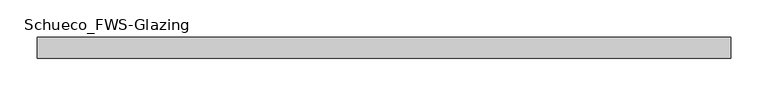
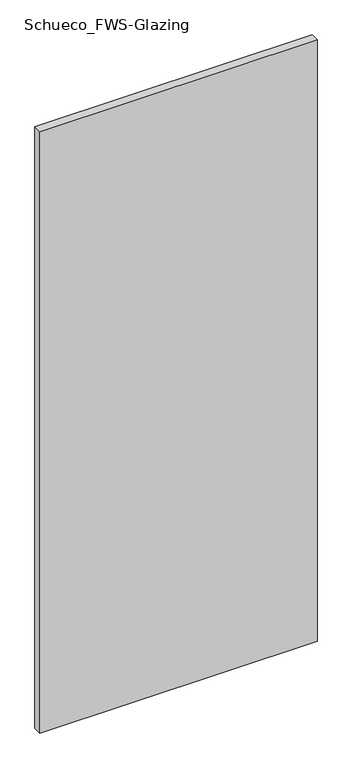
"""IFC4 building model written with IfcOpenShell, lengths in millimetres: plate geometry, Schueco_FWS-Glazing : HI_28mm_DoubGlz."""

from ifc_helpers import new_model, si_unit, origin, origin_with_axes, place, context, project, spatial, polyline, outline, extrude, source, transform, mapped, element, save


def schueco_fws_glazing_3bf565c2(model_context):
    return source(origin(), model_context, "Body", "SweptSolid", [
        extrude(outline(polyline([(464.0, -28.0), (-464.0, -28.0), (-464.0, 0.0), (464.0, 0.0), (464.0, -28.0)])), origin_with_axes(), (0.0, 0.0, 1.0), 2128.0),
    ])


if __name__ == "__main__":
    model = new_model("IFC4")
    model_context = context("Model", 3, world=origin())
    ifc_project = project(units=[si_unit("LENGTHUNIT", "METRE", prefix="MILLI")], contexts=[model_context])
    site = spatial("IfcSite", under=ifc_project)
    building = spatial("IfcBuilding", under=site)
    placement = place(None, origin())
    schueco_fws_glazing_shape = schueco_fws_glazing_3bf565c2(model_context)
    element("IfcPlate", 1, ObjectType="Schueco_FWS-Glazing : HI_28mm_DoubGlz", at=placement, inside=building, context=model_context, shape_type="MappedRepresentation", body=[
        mapped(schueco_fws_glazing_shape, transform((0.0, 0.0, 0.0), x_axis=(1.0, 0.0, 0.0), y_axis=(0.0, 1.0, 0.0), z_axis=(0.0, 0.0, 1.0))),
    ])
    save(model, "model.ifc")

# Revit data of these elements
# Type "Schueco_FWS-Glazing : HI_28mm_DoubGlz"
#   Model = "Double glazing 28mm"
#   Manufacturer = "Schueco International KG"
#   Analytic Construction = "<Keine Auswahl>"
#   Glazing thickness = 28 mm
#   FWS SI insert unit = no
#   FWS HI insert unit = yes
#   Glass = Glass
# Element 1 (IfcPlate, "Schueco_FWS-Glazing : HI_28mm_DoubGlz")
#   Materials on its faces: "Glass"
# Materials
#   "Glass": class "Glass", colour RGB 128 128 255, transparency 0.75, Description = "Soda Lime Glass", Cost = 0
